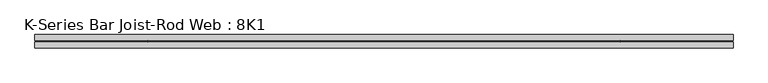
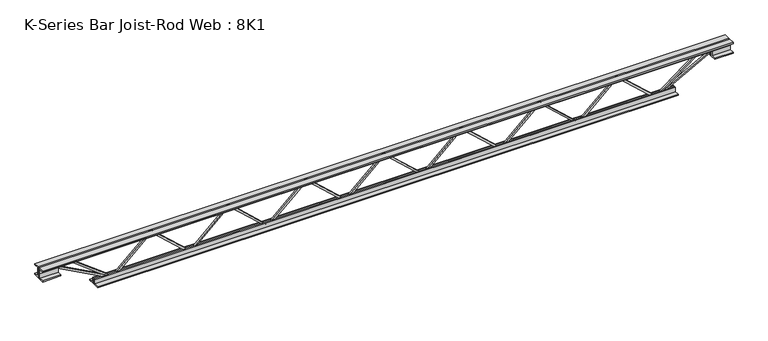
"""IFC4 building model written with IfcOpenShell, lengths in millimetres: beam geometry, K-Series Bar Joist-Rod Web : 8K1."""

from ifc_helpers import new_model, si_unit, frame, origin, place, context, project, spatial, polyline, outline, extrude, source, transform, mapped, element, save


def k_series_bar_joist_rod_web_8k1_8956f8d8(model_context):
    return source(origin(), model_context, "Body", "SweptSolid", [
        extrude(outline(polyline([(-90.4875, 644.6574045), (-100.0125, 644.6574045), (-100.0125, 649.6802342), (90.4875, 858.2160357), (90.4875, 860.8703764), (-100.0125, 1069.4061779), (-100.0125, 1074.4290076), (-90.4875, 1074.4290076), (-90.4875, 1073.1018372), (100.0125, 864.5660357), (100.0125, 854.5203764), (-90.4875, 645.9845749), (-90.4875, 644.6574045)])), frame((0.0, -4.7625, 0.0), z_axis=(0.0, 1.0, 0.0), x_axis=(0.0, 0.0, 1.0)), (0.0, 0.0, 1.0), 9.525),
        extrude(outline(polyline([(-90.4875, 214.8858015), (-100.0125, 214.8858015), (-100.0125, 219.9086312), (90.4875, 428.4444327), (90.4875, 431.0987734), (-100.0125, 639.6345749), (-100.0125, 644.6574045), (-90.4875, 644.6574045), (-90.4875, 643.3302342), (100.0125, 434.7944327), (100.0125, 424.7487734), (-90.4875, 216.2129719), (-90.4875, 214.8858015)])), frame((0.0, -4.7625, 0.0), z_axis=(0.0, 1.0, 0.0), x_axis=(0.0, 0.0, 1.0)), (0.0, 0.0, 1.0), 9.525),
        extrude(outline(polyline([(-90.4875, -214.8858015), (-100.0125, -214.8858015), (-100.0125, -209.8629719), (90.4875, -1.3271704), (90.4875, 1.3271704), (-100.0125, 209.8629719), (-100.0125, 214.8858015), (-90.4875, 214.8858015), (-90.4875, 213.5586312), (100.0125, 5.0228296), (100.0125, -5.0228296), (-90.4875, -213.5586312), (-90.4875, -214.8858015)])), frame((0.0, -4.7625, 0.0), z_axis=(0.0, 1.0, 0.0), x_axis=(0.0, 0.0, 1.0)), (0.0, 0.0, 1.0), 9.525),
        extrude(outline(polyline([(-90.4875, -644.6574045), (-100.0125, -644.6574045), (-100.0125, -639.6345749), (90.4875, -431.0987734), (90.4875, -428.4444327), (-100.0125, -219.9086312), (-100.0125, -214.8858015), (-90.4875, -214.8858015), (-90.4875, -216.2129719), (100.0125, -424.7487734), (100.0125, -434.7944327), (-90.4875, -643.3302342), (-90.4875, -644.6574045)])), frame((0.0, -4.7625, 0.0), z_axis=(0.0, 1.0, 0.0), x_axis=(0.0, 0.0, 1.0)), (0.0, 0.0, 1.0), 9.525),
        extrude(outline(polyline([(-90.4875, -1074.4290076), (-100.0125, -1074.4290076), (-100.0125, -1069.4061779), (90.4875, -860.8703764), (90.4875, -858.2160357), (-100.0125, -649.6802342), (-100.0125, -644.6574045), (-90.4875, -644.6574045), (-90.4875, -645.9845749), (100.0125, -854.5203764), (100.0125, -864.5660357), (-90.4875, -1073.1018372), (-90.4875, -1074.4290076)])), frame((0.0, -4.7625, 0.0), z_axis=(0.0, 1.0, 0.0), x_axis=(0.0, 0.0, 1.0)), (0.0, 0.0, 1.0), 9.525),
        extrude(outline(polyline([(-90.4875, 1074.4290076), (-100.0125, 1074.4290076), (-100.0125, 1079.4518372), (90.4875, 1287.9876387), (90.4875, 1290.6419794), (-100.0125, 1499.1777809), (-100.0125, 1504.2006106), (-90.4875, 1504.2006106), (-90.4875, 1502.8734402), (100.0125, 1294.3376387), (100.0125, 1284.2919794), (-90.4875, 1075.7561779), (-90.4875, 1074.4290076)])), frame((0.0, -4.7625, 0.0), z_axis=(0.0, 1.0, 0.0), x_axis=(0.0, 0.0, 1.0)), (0.0, 0.0, 1.0), 9.525),
        extrude(outline(polyline([(-90.4875, -1504.2006106), (-100.0125, -1504.2006106), (-100.0125, -1499.1777809), (90.4875, -1290.6419794), (90.4875, -1287.9876387), (-100.0125, -1079.4518372), (-100.0125, -1074.4290076), (-90.4875, -1074.4290076), (-90.4875, -1075.7561779), (100.0125, -1284.2919794), (100.0125, -1294.3376387), (-90.4875, -1502.8734402), (-90.4875, -1504.2006106)])), frame((0.0, -4.7625, 0.0), z_axis=(0.0, 1.0, 0.0), x_axis=(0.0, 0.0, 1.0)), (0.0, 0.0, 1.0), 9.525),
        extrude(outline(polyline([(4.7625, 101.6), (36.5125, 101.6), (36.5125, 95.25), (11.1125, 95.25), (11.1125, 69.85), (4.7625, 69.85), (4.7625, 101.6)])), frame((-1910.6006106, 0.0, 0.0), z_axis=(1.0, 0.0, 0.0), x_axis=(0.0, 1.0, 0.0)), (0.0, 0.0, 1.0), 3821.2012212),
        extrude(outline(polyline([(-4.7625, 101.6), (-4.7625, 69.85), (-11.1125, 69.85), (-11.1125, 95.25), (-36.5125, 95.25), (-36.5125, 101.6), (-4.7625, 101.6)])), frame((-1910.6006106, 0.0, 0.0), z_axis=(1.0, 0.0, 0.0), x_axis=(0.0, 1.0, 0.0)), (0.0, 0.0, 1.0), 3821.2012212),
        extrude(outline(polyline([(-4.7625, 38.1), (-36.5125, 38.1), (-36.5125, 44.45), (-11.1125, 44.45), (-11.1125, 69.85), (-4.7625, 69.85), (-4.7625, 38.1)])), frame((-1910.6006106, 0.0, 0.0), z_axis=(1.0, 0.0, 0.0), x_axis=(0.0, 1.0, 0.0)), (0.0, 0.0, 1.0), 101.6),
        extrude(outline(polyline([(36.5125, 38.1), (4.7625, 38.1), (4.7625, 69.85), (11.1125, 69.85), (11.1125, 44.45), (36.5125, 44.45), (36.5125, 38.1)])), frame((-1910.6006106, 0.0, 0.0), z_axis=(1.0, 0.0, 0.0), x_axis=(0.0, 1.0, 0.0)), (0.0, 0.0, 1.0), 101.6),
        extrude(outline(polyline([(4.7625, 38.1), (4.7625, 69.85), (11.1125, 69.85), (11.1125, 44.45), (36.5125, 44.45), (36.5125, 38.1), (4.7625, 38.1)])), frame((1809.0006106, 0.0, 0.0), z_axis=(1.0, 0.0, 0.0), x_axis=(0.0, 1.0, 0.0)), (0.0, 0.0, 1.0), 101.6),
        extrude(outline(polyline([(-4.7625, 38.1), (-36.5125, 38.1), (-36.5125, 44.45), (-11.1125, 44.45), (-11.1125, 69.85), (-4.7625, 69.85), (-4.7625, 38.1)])), frame((1809.0006106, 0.0, 0.0), z_axis=(1.0, 0.0, 0.0), x_axis=(0.0, 1.0, 0.0)), (0.0, 0.0, 1.0), 101.6),
        extrude(outline(polyline([(4.7625, -101.6), (4.7625, -69.85), (11.1125, -69.85), (11.1125, -95.25), (36.5125, -95.25), (36.5125, -101.6), (4.7625, -101.6)])), frame((-1605.8006106, 0.0, 0.0), z_axis=(1.0, 0.0, 0.0), x_axis=(0.0, 1.0, 0.0)), (0.0, 0.0, 1.0), 3211.6012212),
        extrude(outline(polyline([(-4.7625, -101.6), (-36.5125, -101.6), (-36.5125, -95.25), (-11.1125, -95.25), (-11.1125, -69.85), (-4.7625, -69.85), (-4.7625, -101.6)])), frame((-1605.8006106, 0.0, 0.0), z_axis=(1.0, 0.0, 0.0), x_axis=(0.0, 1.0, 0.0)), (0.0, 0.0, 1.0), 3211.6012212),
        extrude(outline(polyline([(0.0, -9.525), (0.0, 0.0), (346.6425392, 0.0), (346.6425392, -9.525), (0.0, -9.525)])), frame((-1811.2689091, 4.7625, 65.662372), z_axis=(0.47628314854008014, 0.0, 0.8792919665371384), x_axis=(0.8792919665371384, 0.0, -0.47628314854008014)), (0.0, 0.0, 1.0), 9.525),
        extrude(outline(polyline([(0.0, -9.525), (0.0, 0.0), (270.9869327, 0.0), (270.9869327, -9.525), (0.0, -9.525)])), frame((-1721.9879865, 4.7625, 66.0734576), z_axis=(0.6092544697894087, 0.0, 0.7929747732693813), x_axis=(0.7929747732693813, 0.0, -0.6092544697894087)), (0.0, 0.0, 1.0), 9.525),
        extrude(outline(polyline([(0.0, -9.525), (0.0, 0.0), (346.6425392, 0.0), (346.6425392, -9.525), (0.0, -9.525)])), frame((1811.2689091, -4.7625, 65.662372), z_axis=(-0.47628314854004167, 0.0, 0.8792919665371591), x_axis=(-0.8792919665371591, 0.0, -0.47628314854004167)), (0.0, 0.0, 1.0), 9.525),
        extrude(outline(polyline([(0.0, -9.525), (0.0, 0.0), (270.9869327, 0.0), (270.9869327, -9.525), (0.0, -9.525)])), frame((1721.9879865, -4.7625, 66.0734576), z_axis=(-0.609254469789387, 0.0, 0.7929747732693979), x_axis=(-0.7929747732693979, 0.0, -0.609254469789387)), (0.0, 0.0, 1.0), 9.525),
    ])


if __name__ == "__main__":
    model = new_model("IFC4")
    model_context = context("Model", 3, world=origin())
    ifc_project = project(units=[si_unit("LENGTHUNIT", "METRE", prefix="MILLI")], contexts=[model_context])
    site = spatial("IfcSite", under=ifc_project)
    building = spatial("IfcBuilding", under=site)
    placement = place(None, origin())
    k_series_bar_joist_rod_web_8k1_shape = k_series_bar_joist_rod_web_8k1_8956f8d8(model_context)
    element("IfcBeam", 1, ObjectType="K-Series Bar Joist-Rod Web : 8K1", at=placement, inside=building, context=model_context, shape_type="MappedRepresentation", body=[
        mapped(k_series_bar_joist_rod_web_8k1_shape, transform((0.0, 0.0, 0.0), x_axis=(1.0, 0.0, 0.0), y_axis=(0.0, 1.0, 0.0), z_axis=(0.0, 0.0, 1.0))),
    ])
    save(model, "model.ifc")

# Revit data of these elements
# Type "K-Series Bar Joist-Rod Web : 8K1"
#   Assembly Code = "B1010350"
#   Wt = 5.1
#   Web Thickness = 0' - 0 3/8"
#   Start Offset [instance default] = 0' - 0"
#   Start Extension [instance default] = 0' - 0"
#   Seat Length = 0' - 4"
#   Seat Depth = 0' - 2 1/2"
#   PanelArrayLength [instance default] = 21' - 4"
#   Panel [instance default] = 1' - 4"
#   End Offset [instance default] = 0' - 0"
#   End Extension [instance default] = 0' - 0"
#   End Panel = 1' - 4"
#   Cord Leg = 0' - 1 1/4"
#   Chord Thickness = 0' - 0 1/4"
#   Length [instance default] = 24' - 0"
#   Depth = 0' - 8"
#   PanelArrayNum [instance default] = 16
#   Rendering Material = none
# Element 1 (IfcBeam, "K-Series Bar Joist-Rod Web : 8K1")
#   PanelArrayLength = 9' - 10.44099"
#   Panel = 1' - 4.92014"
#   PanelArrayNum = 7
